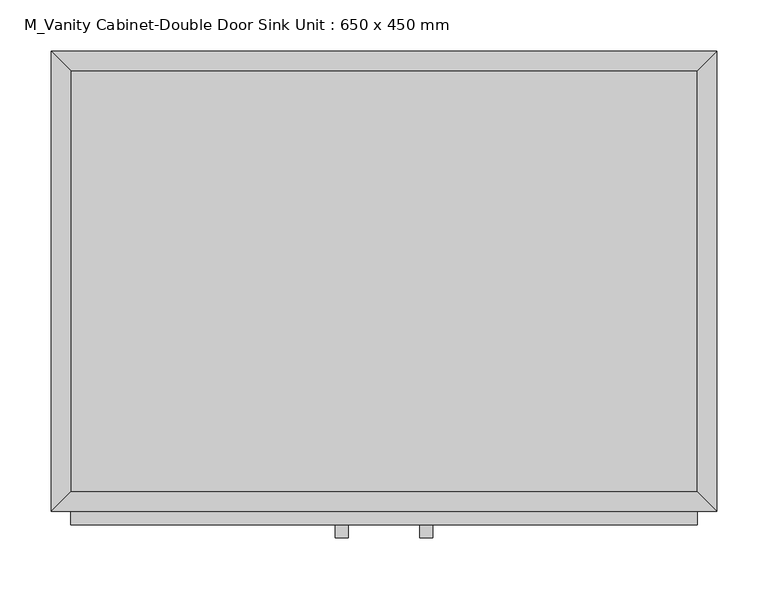
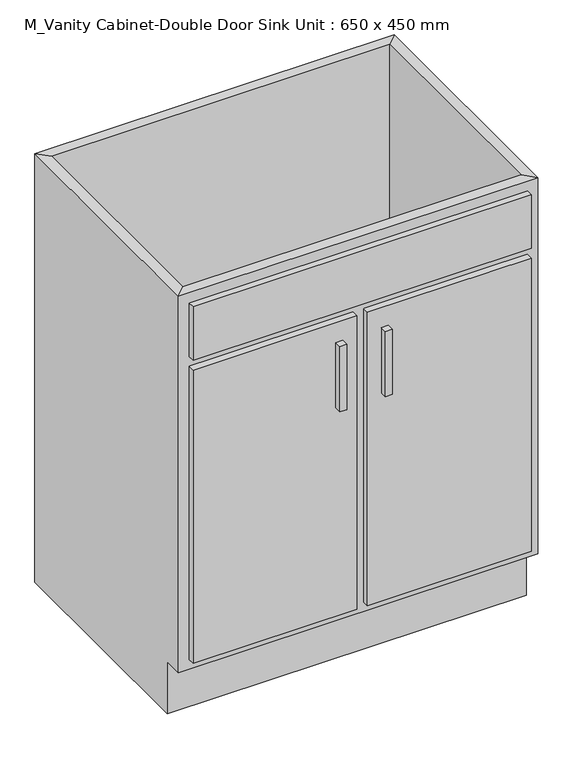
"""IFC4 building model written with IfcOpenShell, lengths in millimetres: furniture geometry, M_Vanity Cabinet-Double Door Sink Unit : 650 x 450 mm."""

from ifc_helpers import new_model, si_unit, frame, origin, place, context, project, spatial, polyline, outline, extrude, faceted_brep, source, transform, mapped, element, save


def m_vanity_cabinet_double_door_sink_unit_650_x_450_mm_a258e0a3(model_context):
    return source(origin(), model_context, "Body", "SolidModel", [
        faceted_brep([(324.6877049, -430.95, 820.0), (324.6877049, -430.95, 100.0), (-287.2122951, -430.95, 100.0), (-287.2122951, -430.95, 820.0), (-306.2622951, -450.0, 820.0), (343.7377049, -450.0, 820.0), (-306.2622951, -450.0, 100.0), (343.7377049, -450.0, 100.0), (-287.2122951, -415.0, 100.0), (-287.2122951, -19.05, 100.0), (-287.2122951, -19.05, 820.0), (-306.2622951, 0.0, 820.0), (-306.2622951, 0.0, 0.0), (-306.2622951, -415.0, 0.0), (-306.2622951, -415.0, 100.0), (324.6877049, -19.05, 100.0), (324.6877049, -19.05, 820.0), (343.7377049, 0.0, 820.0), (343.7377049, 0.0, 0.0), (324.6877049, -415.0, 100.0), (343.7377049, -415.0, 100.0), (343.7377049, -415.0, 0.0)], [[[0, 1, 2, 3]], [[0, 3, 4, 5]], [[5, 4, 6, 7]], [[2, 1, 7, 6]], [[3, 2, 8, 9, 10]], [[4, 3, 10, 11]], [[6, 4, 11, 12, 13, 14]], [[2, 6, 14, 8]], [[10, 9, 15, 16]], [[11, 10, 16, 17]], [[12, 11, 17, 18]], [[1, 0, 16, 15, 19]], [[0, 5, 17, 16]], [[5, 7, 20, 21, 18, 17]], [[7, 1, 19, 20]], [[8, 19, 15, 9]], [[18, 21, 13, 12]], [[13, 21, 20, 19, 8, 14]]]),
        extrude(outline(polyline([(-16.1872951, -475.4), (-28.8872951, -475.4), (-28.8872951, -462.7), (-16.1872951, -462.7), (-16.1872951, -475.4)])), frame((0.0, 0.0, 517.469895), z_axis=(0.0, 0.0, 1.0), x_axis=(1.0, 0.0, 0.0)), (0.0, 0.0, 1.0), 124.730105),
        extrude(outline(polyline([(66.3627049, -475.4), (53.6627049, -475.4), (53.6627049, -462.7), (66.3627049, -462.7), (66.3627049, -475.4)])), frame((0.0, 0.0, 517.469895), z_axis=(0.0, 0.0, 1.0), x_axis=(1.0, 0.0, 0.0)), (0.0, 0.0, 1.0), 124.730105),
        extrude(outline(polyline([(9.2127049, -462.7), (-287.2122951, -462.7), (-287.2122951, -450.0), (9.2127049, -450.0), (9.2127049, -462.7)])), frame((0.0, 0.0, 119.05), z_axis=(0.0, 0.0, 1.0), x_axis=(1.0, 0.0, 0.0)), (0.0, 0.0, 1.0), 561.25),
        extrude(outline(polyline([(324.6877049, -462.7), (28.2627049, -462.7), (28.2627049, -450.0), (324.6877049, -450.0), (324.6877049, -462.7)])), frame((0.0, 0.0, 119.05), z_axis=(0.0, 0.0, 1.0), x_axis=(1.0, 0.0, 0.0)), (0.0, 0.0, 1.0), 561.25),
        extrude(outline(polyline([(324.6877049, -462.7), (-287.2122951, -462.7), (-287.2122951, -450.0), (324.6877049, -450.0), (324.6877049, -462.7)])), frame((0.0, 0.0, 699.35), z_axis=(0.0, 0.0, 1.0), x_axis=(1.0, 0.0, 0.0)), (0.0, 0.0, 1.0), 101.6),
        extrude(outline(polyline([(324.6877049, -19.05), (324.6877049, -430.95), (-287.2122951, -430.95), (-287.2122951, -19.05), (324.6877049, -19.05)])), frame((0.0, 0.0, 100.0), z_axis=(0.0, 0.0, 1.0), x_axis=(1.0, 0.0, 0.0)), (0.0, 0.0, 1.0), 19.05),
    ])


if __name__ == "__main__":
    model = new_model("IFC4")
    model_context = context("Model", 3, world=origin())
    ifc_project = project(units=[si_unit("LENGTHUNIT", "METRE", prefix="MILLI")], contexts=[model_context])
    site = spatial("IfcSite", under=ifc_project)
    building = spatial("IfcBuilding", under=site)
    placement = place(None, origin())
    m_vanity_cabinet_double_door_sink_unit_650_x_450_mm_shape = m_vanity_cabinet_double_door_sink_unit_650_x_450_mm_a258e0a3(model_context)
    element("IfcFurniture", 1, ObjectType="M_Vanity Cabinet-Double Door Sink Unit : 650 x 450 mm", at=placement, inside=building, context=model_context, shape_type="MappedRepresentation", body=[
        mapped(m_vanity_cabinet_double_door_sink_unit_650_x_450_mm_shape, transform((0.0, 0.0, 0.0), x_axis=(1.0, 0.0, 0.0), y_axis=(0.0, 1.0, 0.0), z_axis=(0.0, 0.0, 1.0))),
    ])
    save(model, "model.ifc")

# Revit data of these elements
# Type "M_Vanity Cabinet-Double Door Sink Unit : 650 x 450 mm"
#   Manufacturer = "Manufacturer"
#   Finish = "Finish"
#   Construction Type = "Construction Type"
#   AccessibilityPerformance = "AccessibilityPerformance"
#   CodePerformance = "CodePerformance"
#   Area = "Area"
#   Color = "Color"
#   Constituents = "Constituents"
#   Features = "Features"
#   Finish = "Finish"
#   Grade = "Grade"
#   Material = "Material"
#   ModelReference = "ModelReference"
#   NominalHeight = "NominalHeight"
#   NominalLength = "NominalLength"
#   NominalWidth = "NominalWidth"
#   ProductionYear = "ProductionYear"
#   Reference = "Reference"
#   Shape = "Shape"
#   Size = "Size"
#   SustainabilityPerformance = "SustainabilityPerformance"
#   WarrantyDescription = "WarrantyDescription"
#   WarrantyDurationLabor = "WarrantyDurationLabor"
#   WarrantyDurationParts = "WarrantyDurationParts"
#   WarrantyGuarantorLabor = "WarrantyGuarantorLabor"
#   WarrantyGuarantorParts = "WarrantyGuarantorParts"
#   ExpectedLife = "ExpectedLife"
#   ReplacementCost = "ReplacementCost"
#   AssetAccountingType = "FIXED"
#   ModelLabel = "ModelLabel"
#   Depth = 0.450 m
#   Height = 0.820 m
#   Plinth Depth = 0.035 m
#   Plinth Height = 0.100 m
#   Width = 0.650 m
#   Cabinet Material = none
#   Door/Drawer Material = none
#   Handle Material = Cabinets - Handles
# Element 1 (IfcFurniture, "M_Vanity Cabinet-Double Door Sink Unit : 650 x 450 mm")
#   Materials on its faces: "Cabinets", "Cabinets - Handles"
# Materials
#   "Cabinets - Handles": class "Metal", colour RGB 57 57 57, transparency 0
#   "Cabinets": class "Miscellaneous", colour RGB 249 249 249, transparency 0
